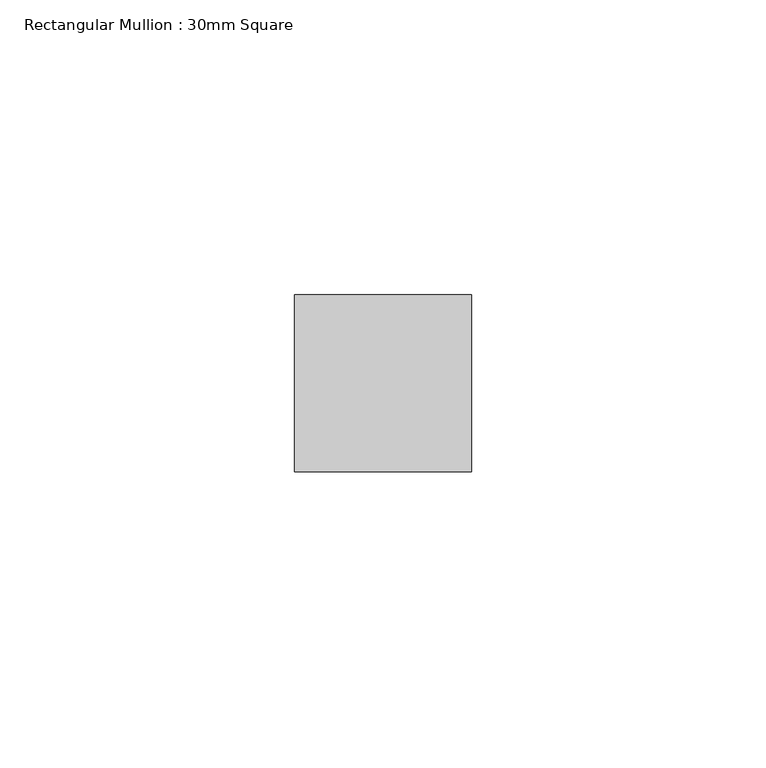
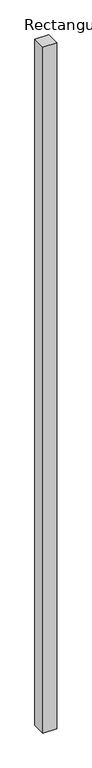
"""IFC4 building model written with IfcOpenShell, lengths in millimetres: member geometry, Rectangular Mullion : 30mm Square."""

from ifc_helpers import new_model, si_unit, frame, origin, place, context, project, spatial, polyline, outline, extrude, source, transform, mapped, element, save


def rectangular_mullion_30mm_square_028e2ba1(model_context):
    return source(origin(), model_context, "Body", "SweptSolid", [
        extrude(outline(polyline([(15.0, 15.0), (15.0, -15.0), (-15.0, -15.0), (-15.0, 15.0), (15.0, 15.0)])), frame((0.0, 0.0, -1571.0515916), z_axis=(0.0, 0.0, 1.0), x_axis=(1.0, 0.0, 0.0)), (0.0, 0.0, 1.0), 1571.0515916),
    ])


if __name__ == "__main__":
    model = new_model("IFC4")
    model_context = context("Model", 3, world=origin())
    ifc_project = project(units=[si_unit("LENGTHUNIT", "METRE", prefix="MILLI")], contexts=[model_context])
    site = spatial("IfcSite", under=ifc_project)
    building = spatial("IfcBuilding", under=site)
    placement = place(None, origin())
    rectangular_mullion_30mm_square_shape = rectangular_mullion_30mm_square_028e2ba1(model_context)
    element("IfcMember", 1, ObjectType="Rectangular Mullion : 30mm Square", at=placement, inside=building, context=model_context, shape_type="MappedRepresentation", body=[
        mapped(rectangular_mullion_30mm_square_shape, transform((0.0, 0.0, 0.0), x_axis=(1.0, 0.0, 0.0), y_axis=(0.0, 1.0, 0.0), z_axis=(0.0, 0.0, 1.0))),
    ])
    save(model, "model.ifc")

# Revit data of these elements
# Type "Rectangular Mullion : 30mm Square"
#   built-in parameter 1007304 = 0.0984252 (stored number, unit not read)
#   built-in parameter 1007301 = 0.0492126 (stored number, unit not read)
#   built-in parameter 1007300 = 0.0492126 (stored number, unit not read)
# Element 1 (IfcMember, "Rectangular Mullion : 30mm Square")
#   Materials on its faces: "Aluminum"
# Materials
#   "Aluminum": class "Metal", colour RGB 244 244 244, transparency 0, Description = "Aluminum 6061", Cost = 0
